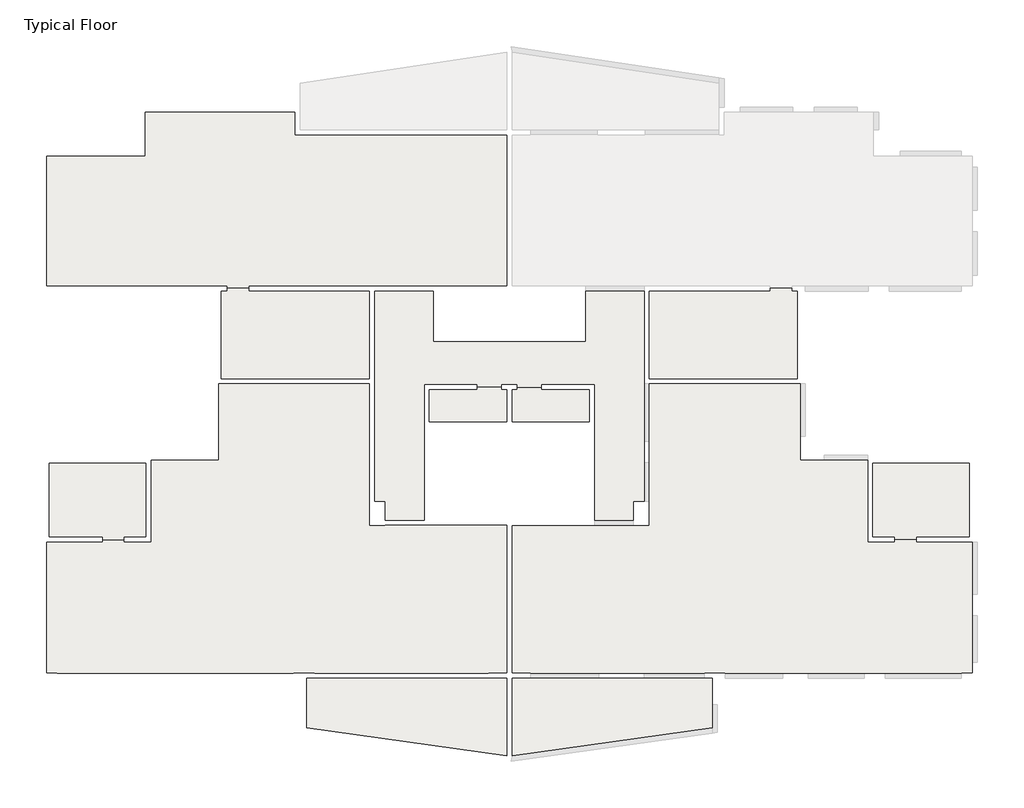
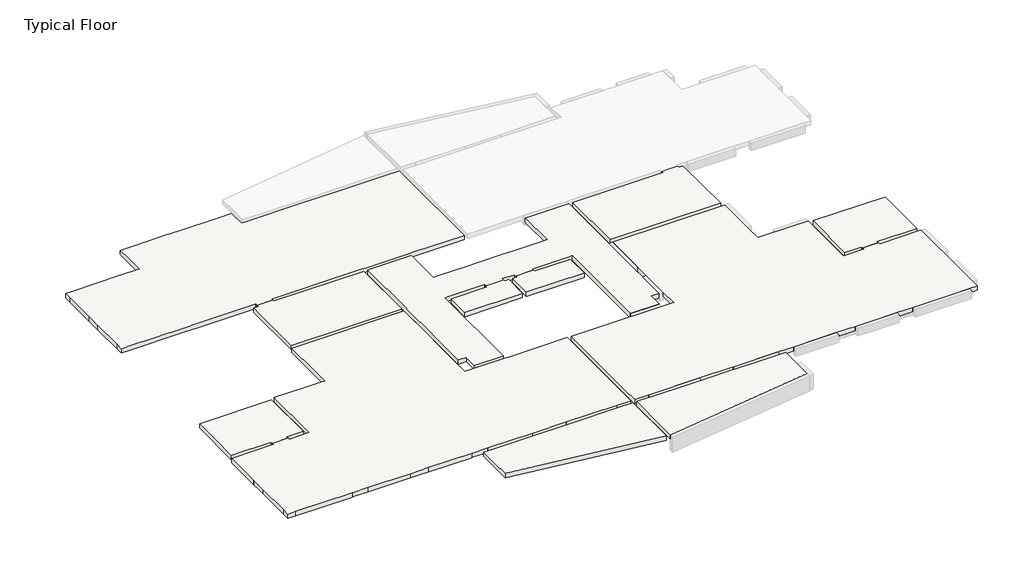
# One storey, part 1 of 2: 12 slabs.
"""IFC4 building model written with IfcOpenShell, lengths in millimetres."""

from ifc_helpers import new_model, si_unit, frame, origin, place, context, project, spatial, polyline, outline, extrude, faceted_brep, element, save

model = new_model("IFC4")

# Units and contexts
model_context = context("Model", 3, world=origin())
ifc_project = project(units=[si_unit("LENGTHUNIT", "METRE", prefix="MILLI")], contexts=[model_context])

# Site, building, storey
site = spatial("IfcSite", under=ifc_project)
building = spatial("IfcBuilding", under=site)
storey = spatial("IfcBuildingStorey", under=building, Name="Typical Floor", Elevation=3120.0)

# Slabs
placement = place(None, origin())
element("IfcSlab", 1, ObjectType="23", at=placement, inside=storey, context=model_context, shape_type="Brep", body=[
    faceted_brep([(-17867.839929, -8104.8146558, 2890.0), (-17867.839929, -8004.8146558, 2890.0), (-17067.8037495, -8004.8146558, 2890.0), (-17067.8037495, -8104.8146558, 2890.0), (-16045.535298, -8104.8146558, 2890.0), (-16045.535298, -7904.8146558, 2890.0), (-16045.535298, -5135.8928035, 2890.0), (-16045.535298, -5036.9600972, 2890.0), (-14415.271188, -5036.9600972, 2890.0), (-13515.271188, -5036.9600972, 2890.0), (-13515.271188, -4136.9600972, 2890.0), (-13515.271188, -2169.1055386, 2890.0), (-7866.3203921, -2169.1055386, 2890.0), (-7866.3023024, -7475.6540191, 2890.0), (-7266.3023024, -7475.6540191, 2890.0), (-7266.3023024, -7475.1655965, 2890.0), (-5816.5012893, -7475.1655965, 2890.0), (-5816.3023024, -7475.1655965, 2890.0), (-5616.5012893, -7475.1655965, 2890.0), (-2716.392751, -7475.1655965, 2890.0), (-2716.392751, -12204.5252202, 2890.0), (-2716.392751, -13004.5252202, 2890.0), (-3416.392751, -13004.5252202, 2890.0), (-3416.392751, -13009.5252202, 2890.0), (-5966.3203921, -13009.5252202, 2890.0), (-5966.3203921, -13005.5744243, 2890.0), (-6816.392751, -13005.5744243, 2890.0), (-7666.3203921, -13005.5744243, 2890.0), (-7666.3203921, -13009.5252202, 2890.0), (-9916.193764, -13009.5252202, 2890.0), (-9916.193764, -13004.5252202, 2890.0), (-10716.193764, -13004.5252202, 2890.0), (-10716.193764, -13009.5252202, 2890.0), (-12866.5555585, -13009.5252202, 2890.0), (-12866.5555585, -13005.8747137, 2890.0), (-13341.5555585, -13005.8747137, 2890.0), (-13816.5555585, -13005.8747137, 2890.0), (-13816.5555585, -13009.5252202, 2890.0), (-15916.4289304, -13009.5252202, 2890.0), (-15916.4289304, -13005.8747137, 2890.0), (-16316.4289304, -13005.8747137, 2890.0), (-16716.4289304, -13005.8747137, 2890.0), (-16716.4289304, -13009.5252202, 2890.0), (-19564.2400737, -13009.5252202, 2890.0), (-19564.2400737, -13004.5252202, 2890.0), (-19964.2400737, -13004.5252202, 2890.0), (-19964.2400737, -12604.5252202, 2890.0), (-19966.2400737, -12604.5252202, 2890.0), (-19966.2400737, -10855.1764503, 2890.0), (-19965.2892778, -10855.1764503, 2890.0), (-19965.2892778, -10455.1764503, 2890.0), (-19965.2892778, -10055.1764503, 2890.0), (-19966.2400737, -10055.1764503, 2890.0), (-19966.2400737, -8105.8819496, 2890.0), (-19964.2400737, -8105.8819496, 2890.0), (-19864.2400737, -8105.8819496, 2890.0), (-19864.2400737, -8104.8146558, 2890.0), (-17867.839929, -8004.8146558, 3120.0), (-17867.839929, -8104.8146558, 3120.0), (-19864.2400737, -8104.8146558, 3120.0), (-19864.2400737, -8105.8819496, 3120.0), (-19966.2400737, -8105.8819496, 3120.0), (-19966.2400737, -10055.1764503, 3120.0), (-19965.2892778, -10055.1764503, 3120.0), (-19965.2892778, -10855.1764503, 3120.0), (-19966.2400737, -10855.1764503, 3120.0), (-19966.2400737, -12604.5252202, 3120.0), (-19964.2400737, -12604.5252202, 3120.0), (-19964.2400737, -13004.5252202, 3120.0), (-19564.2400737, -13004.5252202, 3120.0), (-19564.2400737, -13009.5252202, 3120.0), (-16716.4289304, -13009.5252202, 3120.0), (-16716.4289304, -13005.8747137, 3120.0), (-15916.4289304, -13005.8747137, 3120.0), (-15916.4289304, -13009.5252202, 3120.0), (-13816.5555585, -13009.5252202, 3120.0), (-13816.5555585, -13005.8747137, 3120.0), (-12866.5555585, -13005.8747137, 3120.0), (-12866.5555585, -13009.5252202, 3120.0), (-10716.193764, -13009.5252202, 3120.0), (-10716.193764, -13004.5252202, 3120.0), (-9916.193764, -13004.5252202, 3120.0), (-9916.193764, -13009.5252202, 3120.0), (-7666.3203921, -13009.5252202, 3120.0), (-7666.3203921, -13005.5744243, 3120.0), (-5966.3203921, -13005.5744243, 3120.0), (-5966.3203921, -13009.5252202, 3120.0), (-3416.392751, -13009.5252202, 3120.0), (-3416.392751, -13004.5252202, 3120.0), (-2716.392751, -13004.5252202, 3120.0), (-2716.392751, -12204.5252202, 3120.0), (-2716.392751, -7475.1655965, 3120.0), (-5616.5012893, -7475.1655965, 3120.0), (-5816.5012893, -7475.1655965, 3120.0), (-7266.3023024, -7475.1655965, 3120.0), (-7266.3023024, -7475.6540191, 3120.0), (-7866.3023024, -7475.6540191, 3120.0), (-7866.3053704, -6575.654019, 3120.0), (-7866.3103273, -5121.5838309, 3120.0), (-7866.3130544, -4321.5838309, 3120.0), (-7866.3203921, -2169.1055386, 3120.0), (-13515.271188, -2169.1055386, 3120.0), (-13515.271188, -4136.9600972, 3120.0), (-13515.271188, -5036.9600972, 3120.0), (-14415.271188, -5036.9600972, 3120.0), (-16045.271188, -5036.9600972, 3120.0), (-16045.535298, -5036.9600972, 3120.0), (-16045.535298, -5135.8928035, 3120.0), (-16045.535298, -7904.8146558, 3120.0), (-16045.535298, -8104.8146558, 3120.0), (-17067.8037495, -8104.8146558, 3120.0), (-17067.8037495, -8004.8146558, 3120.0)], [[[0, 1, 2, 3, 4, 5, 6, 7, 8, 9, 10, 11, 12, 13, 14, 15, 16, 17, 18, 19, 20, 21, 22, 23, 24, 25, 26, 27, 28, 29, 30, 31, 32, 33, 34, 35, 36, 37, 38, 39, 40, 41, 42, 43, 44, 45, 46, 47, 48, 49, 50, 51, 52, 53, 54, 55, 56]], [[57, 58, 59, 60, 61, 62, 63, 64, 65, 66, 67, 68, 69, 70, 71, 72, 73, 74, 75, 76, 77, 78, 79, 80, 81, 82, 83, 84, 85, 86, 87, 88, 89, 90, 91, 92, 93, 94, 95, 96, 97, 98, 99, 100, 101, 102, 103, 104, 105, 106, 107, 108, 109, 110, 111]], [[12, 100, 99, 98, 97, 96, 13]], [[91, 19, 18, 17, 16, 15, 94, 93, 92]], [[19, 91, 90, 89, 21, 20]], [[23, 87, 86, 24]], [[82, 29, 28, 83]], [[32, 79, 78, 33]], [[70, 43, 42, 71]], [[74, 38, 37, 75]], [[47, 66, 65, 48]], [[61, 53, 52, 62]], [[58, 0, 56, 59]], [[1, 0, 58, 57]], [[2, 1, 57, 111]], [[3, 2, 111, 110]], [[4, 3, 110, 109]], [[4, 109, 108, 107, 106, 7, 6, 5]], [[7, 106, 105, 104, 103, 9, 8]], [[9, 103, 102, 101, 11, 10]], [[12, 11, 101, 100]], [[22, 88, 87, 23]], [[88, 22, 21, 89]], [[31, 80, 79, 32]], [[80, 31, 30, 81]], [[81, 30, 29, 82]], [[46, 67, 66, 47]], [[45, 68, 67, 46]], [[68, 45, 44, 69]], [[69, 44, 43, 70]], [[14, 95, 94, 15]], [[95, 14, 13, 96]], [[55, 60, 59, 56]], [[60, 55, 54, 53, 61]], [[49, 64, 63, 51, 50]], [[64, 49, 48, 65]], [[51, 63, 62, 52]], [[39, 73, 72, 41, 40]], [[73, 39, 38, 74]], [[41, 72, 71, 42]], [[34, 77, 76, 36, 35]], [[77, 34, 33, 78]], [[36, 76, 75, 37]], [[25, 85, 84, 27, 26]], [[85, 25, 24, 86]], [[27, 84, 83, 28]]]),
])
element("IfcSlab", 2, ObjectType="23", at=placement, inside=storey, context=model_context, shape_type="SweptSolid", body=[
    extrude(outline(polyline([(-16245.535298, -5135.8928035), (-16245.535298, -7904.8146558), (-17067.8037495, -7904.8146558), (-17067.8037495, -8004.8146558), (-17867.839929, -8004.8146558), (-17867.839929, -7904.8146558), (-19864.2400737, -7904.8146558), (-19864.2400737, -5135.8928035), (-16245.535298, -5135.8928035)])), frame((0.0, 0.0, 2890.0), z_axis=(0.0, 0.0, 1.0), x_axis=(1.0, 0.0, 0.0)), (0.0, 0.0, 1.0), 230.0),
])
element("IfcSlab", 3, ObjectType="23", at=placement, inside=storey, context=model_context, shape_type="Brep", body=[
    faceted_brep([(-2716.392751, -13204.5252202, 2890.0), (-2716.392751, -16112.674045, 2890.0), (-10216.193764, -15058.6457505, 2890.0), (-10216.193764, -14204.5252202, 2890.0), (-10216.193764, -13204.5252202, 2890.0), (-9916.193764, -13204.5252202, 2890.0), (-7666.3203921, -13204.5252202, 2890.0), (-7666.3203921, -13205.5744243, 2890.0), (-5966.3203921, -13205.5744243, 2890.0), (-5966.3203921, -13204.5252202, 2890.0), (-2716.392751, -16112.674045, 3120.0), (-2716.392751, -13204.5252202, 3120.0), (-3416.392751, -13204.5252202, 3120.0), (-5966.3203921, -13204.5252202, 3120.0), (-5966.3203921, -13205.5744243, 3120.0), (-7666.3203921, -13205.5744243, 3120.0), (-7666.3203921, -13204.5252202, 3120.0), (-9916.193764, -13204.5252202, 3120.0), (-10216.193764, -13204.5252202, 3120.0), (-10216.193764, -14204.5252202, 3120.0), (-10216.193764, -15058.6457505, 3120.0)], [[[0, 1, 2, 3, 4, 5, 6, 7, 8, 9]], [[10, 11, 12, 13, 14, 15, 16, 17, 18, 19, 20]], [[1, 0, 11, 10]], [[2, 1, 10, 20]], [[2, 20, 19, 18, 4, 3]], [[11, 0, 9, 13, 12]], [[4, 18, 17, 16, 6, 5]], [[8, 14, 13, 9]], [[14, 8, 7, 15]], [[15, 7, 6, 16]]]),
])
element("IfcSlab", 4, ObjectType="23", at=placement, inside=storey, context=model_context, shape_type="Brep", body=[
    faceted_brep([(-12396.6930404, 1513.6006842, 2890.0), (-12396.6930404, 1413.6006842, 2890.0), (-13195.271188, 1413.6006842, 2890.0), (-13196.6930404, 1413.6006842, 2890.0), (-13196.6930404, 1514.1252863, 2890.0), (-13715.271188, 1514.1252863, 2890.0), (-16062.5034601, 1514.1252863, 2890.0), (-16862.5034601, 1514.1252863, 2890.0), (-19564.2400737, 1514.1252863, 2890.0), (-19964.2400737, 1514.1252863, 2890.0), (-19964.2400737, 1914.1252863, 2890.0), (-19969.2400737, 1914.1252863, 2890.0), (-19969.2400737, 3539.1252863, 2890.0), (-19965.2892778, 3539.1252863, 2890.0), (-19965.2892778, 3934.6498883, 2890.0), (-19965.2892778, 4339.1252863, 2890.0), (-19969.2400737, 4339.1252863, 2890.0), (-19969.2400737, 5963.5645048, 2890.0), (-19964.2400737, 5963.5645048, 2890.0), (-19964.2400737, 6363.5645048, 2890.0), (-19564.2400737, 6363.5645048, 2890.0), (-17264.6018682, 6363.5645048, 2890.0), (-16264.6018682, 6363.5645048, 2890.0), (-16264.6018682, 7363.5645048, 2890.0), (-16264.6018682, 8012.3163138, 2890.0), (-11266.4470202, 8012.3163138, 2890.0), (-10666.4470202, 8012.3163138, 2890.0), (-10666.4470202, 7162.3163138, 2890.0), (-10466.4470202, 7162.3163138, 2890.0), (-10466.4470202, 7163.6006842, 2890.0), (-10466.4470202, 7163.7694287, 2890.0), (-7705.3941982, 7163.7694287, 2890.0), (-7705.3941982, 7163.6006842, 2890.0), (-5905.3941982, 7163.6006842, 2890.0), (-5905.3941982, 7163.7694287, 2890.0), (-3416.392751, 7163.7694287, 2890.0), (-3416.392751, 7163.6006842, 2890.0), (-2716.392751, 7163.6006842, 2890.0), (-2716.392751, 6363.6006842, 2890.0), (-2716.392751, 1513.6006842, 2890.0), (-5279.9781345, 1513.6006842, 2890.0), (-5479.9781345, 1513.6006842, 2890.0), (-7666.3203921, 1513.6006842, 2890.0), (-7866.3203921, 1513.6006842, 2890.0), (-12396.6930404, 1413.6006842, 3120.0), (-12396.6930404, 1513.6006842, 3120.0), (-7866.3203921, 1513.6006842, 3120.0), (-7666.3203921, 1513.6006842, 3120.0), (-5479.9781345, 1513.6006842, 3120.0), (-5279.9781345, 1513.6006842, 3120.0), (-2716.392751, 1513.6006842, 3120.0), (-2716.392751, 6363.6006842, 3120.0), (-2716.392751, 7163.6006842, 3120.0), (-3416.392751, 7163.6006842, 3120.0), (-3416.392751, 7163.7694287, 3120.0), (-5905.3941982, 7163.7694287, 3120.0), (-5905.3941982, 7163.6006842, 3120.0), (-7705.3941982, 7163.6006842, 3120.0), (-7705.3941982, 7163.7694287, 3120.0), (-10466.4470202, 7163.7694287, 3120.0), (-10466.4470202, 7162.3163138, 3120.0), (-10666.4470202, 7162.3163138, 3120.0), (-10666.4470202, 8012.3163138, 3120.0), (-11266.4470202, 8012.3163138, 3120.0), (-13239.0953559, 8012.3163138, 3120.0), (-14039.0953559, 8012.3163138, 3120.0), (-15664.5656888, 8012.3163138, 3120.0), (-16264.6018682, 8012.3163138, 3120.0), (-16264.6018682, 7363.5645048, 3120.0), (-16264.6018682, 6363.5645048, 3120.0), (-17264.6018682, 6363.5645048, 3120.0), (-19564.2400737, 6363.5645048, 3120.0), (-19964.2400737, 6363.5645048, 3120.0), (-19964.2400737, 5963.5645048, 3120.0), (-19969.2400737, 5963.5645048, 3120.0), (-19969.2400737, 4339.1252863, 3120.0), (-19965.2892778, 4339.1252863, 3120.0), (-19965.2892778, 3539.1252863, 3120.0), (-19969.2400737, 3539.1252863, 3120.0), (-19969.2400737, 1914.1252863, 3120.0), (-19964.2400737, 1914.1252863, 3120.0), (-19964.2400737, 1514.1252863, 3120.0), (-19564.2400737, 1514.1252863, 3120.0), (-16862.5034601, 1514.1252863, 3120.0), (-16062.5034601, 1514.1252863, 3120.0), (-13715.271188, 1514.1252863, 3120.0), (-13196.6930404, 1514.1252863, 3120.0), (-13196.6930404, 1413.6006842, 3120.0), (-13195.271188, 1413.6006842, 3120.0)], [[[0, 1, 2, 3, 4, 5, 6, 7, 8, 9, 10, 11, 12, 13, 14, 15, 16, 17, 18, 19, 20, 21, 22, 23, 24, 25, 26, 27, 28, 29, 30, 31, 32, 33, 34, 35, 36, 37, 38, 39, 40, 41, 42, 43]], [[44, 45, 46, 47, 48, 49, 50, 51, 52, 53, 54, 55, 56, 57, 58, 59, 60, 61, 62, 63, 64, 65, 66, 67, 68, 69, 70, 71, 72, 73, 74, 75, 76, 77, 78, 79, 80, 81, 82, 83, 84, 85, 86, 87, 88]], [[26, 62, 61, 27]], [[30, 59, 58, 31]], [[54, 35, 34, 55]], [[50, 39, 38, 37, 52, 51]], [[39, 50, 49, 48, 47, 46, 45, 0, 43, 42, 41, 40]], [[1, 0, 45, 44]], [[3, 2, 1, 44, 88, 87]], [[4, 3, 87, 86]], [[4, 86, 85, 84, 83, 82, 81, 9, 8, 7, 6, 5]], [[11, 79, 78, 12]], [[74, 17, 16, 75]], [[69, 22, 21, 20, 19, 72, 71, 70]], [[22, 69, 68, 67, 24, 23]], [[24, 67, 66, 65, 64, 63, 62, 26, 25]], [[36, 53, 52, 37]], [[53, 36, 35, 54]], [[10, 80, 79, 11]], [[80, 10, 9, 81]], [[18, 73, 72, 19]], [[73, 18, 17, 74]], [[28, 60, 59, 30, 29]], [[27, 61, 60, 28]], [[33, 56, 55, 34]], [[56, 33, 32, 57]], [[57, 32, 31, 58]], [[15, 76, 75, 16]], [[76, 15, 14, 13, 77]], [[77, 13, 12, 78]]]),
])
element("IfcSlab", 5, ObjectType="23", at=placement, inside=storey, context=model_context, shape_type="SweptSolid", body=[
    extrude(outline(polyline([(-7866.3203921, -1969.1055386), (-13415.271188, -1969.1055386), (-13415.271188, 1313.6006842), (-13195.271188, 1313.6006842), (-13195.271188, 1413.6006842), (-12396.6930404, 1413.6006842), (-12396.6930404, 1313.6006842), (-7866.3203921, 1313.6006842), (-7866.3203921, -1969.1055386)])), frame((0.0, 0.0, 2890.0), z_axis=(0.0, 0.0, 1.0), x_axis=(1.0, 0.0, 0.0)), (0.0, 0.0, 1.0), 230.0),
])
element("IfcSlab", 6, ObjectType="23", at=placement, inside=storey, context=model_context, shape_type="Brep", body=[
    faceted_brep([(11835.0182476, -8004.8146558, 2890.0), (12635.054427, -8004.8146558, 2890.0), (12635.054427, -8104.8146558, 2890.0), (14631.4545717, -8104.8146558, 2890.0), (14631.4545717, -8105.8819496, 2890.0), (14731.4545717, -8105.8819496, 2890.0), (14731.4545717, -12604.5252202, 2890.0), (14731.4545717, -13004.5252202, 2890.0), (14331.4545717, -13004.5252202, 2890.0), (14331.4545717, -13009.5252202, 2890.0), (11483.6434285, -13009.5252202, 2890.0), (11483.6434285, -13005.8747137, 2890.0), (11083.6434285, -13005.8747137, 2890.0), (10683.6434285, -13005.8747137, 2890.0), (10683.6434285, -13009.5252202, 2890.0), (8583.7700565, -13009.5252202, 2890.0), (8583.7700565, -13005.8747137, 2890.0), (8108.7700565, -13005.8747137, 2890.0), (7633.7700565, -13005.8747137, 2890.0), (7633.7700565, -13009.5252202, 2890.0), (5483.408262, -13009.5252202, 2890.0), (5483.408262, -13004.5252202, 2890.0), (4683.408262, -13004.5252202, 2890.0), (4683.408262, -13009.5252202, 2890.0), (2433.5348901, -13009.5252202, 2890.0), (2433.5348901, -13005.5744243, 2890.0), (1583.607249, -13005.5744243, 2890.0), (733.5348901, -13005.5744243, 2890.0), (733.5348901, -13009.5252202, 2890.0), (-1816.392751, -13009.5252202, 2890.0), (-1816.392751, -13004.5252202, 2890.0), (-2516.392751, -13004.5252202, 2890.0), (-2516.392751, -12204.5252202, 2890.0), (-2516.392751, -7475.6540191, 2890.0), (2033.5168004, -7475.6540191, 2890.0), (2633.5348901, -7475.6540191, 2890.0), (2633.5348901, -6575.6540191, 2890.0), (2633.5348901, -5121.583831, 2890.0), (2633.5348901, -4321.583831, 2890.0), (2633.5348901, -2169.1055386, 2890.0), (8282.4856861, -2169.1055386, 2890.0), (8282.4856861, -4136.9600972, 2890.0), (8282.4856861, -5036.9600972, 2890.0), (9182.4856861, -5036.9600972, 2890.0), (10812.749796, -5036.9600972, 2890.0), (10812.749796, -5135.8928035, 2890.0), (10812.749796, -7904.8146558, 2890.0), (10812.749796, -8104.8146558, 2890.0), (11835.0182476, -8104.8146558, 2890.0), (12635.054427, -8004.8146558, 3120.0), (11835.0182476, -8004.8146558, 3120.0), (11835.0182476, -8104.8146558, 3120.0), (10812.749796, -8104.8146558, 3120.0), (10812.749796, -7904.8146558, 3120.0), (10812.749796, -5135.8928035, 3120.0), (10812.749796, -5036.9600972, 3120.0), (10812.4856861, -5036.9600972, 3120.0), (9182.4856861, -5036.9600972, 3120.0), (8282.4856861, -5036.9600972, 3120.0), (8282.4856861, -4136.9600972, 3120.0), (8282.4856861, -2169.1055386, 3120.0), (2633.5348901, -2169.1055386, 3120.0), (2633.5348901, -4321.583831, 3120.0), (2633.5348901, -5121.583831, 3120.0), (2633.5348901, -6575.6540191, 3120.0), (2633.5348901, -7475.6540191, 3120.0), (2033.5168004, -7475.6540191, 3120.0), (583.5168004, -7475.6540191, 3120.0), (-2516.392751, -7475.6540191, 3120.0), (-2516.392751, -12204.5252202, 3120.0), (-2516.392751, -13004.5252202, 3120.0), (-1816.392751, -13004.5252202, 3120.0), (-1816.392751, -13009.5252202, 3120.0), (733.5348901, -13009.5252202, 3120.0), (733.5348901, -13005.5744243, 3120.0), (2433.5348901, -13005.5744243, 3120.0), (2433.5348901, -13009.5252202, 3120.0), (4683.408262, -13009.5252202, 3120.0), (4683.408262, -13004.5252202, 3120.0), (5483.408262, -13004.5252202, 3120.0), (5483.408262, -13009.5252202, 3120.0), (7633.7700565, -13009.5252202, 3120.0), (7633.7700565, -13005.8747137, 3120.0), (8583.7700565, -13005.8747137, 3120.0), (8583.7700565, -13009.5252202, 3120.0), (10683.6434285, -13009.5252202, 3120.0), (10683.6434285, -13005.8747137, 3120.0), (11483.6434285, -13005.8747137, 3120.0), (11483.6434285, -13009.5252202, 3120.0), (14331.4545717, -13009.5252202, 3120.0), (14331.4545717, -13004.5252202, 3120.0), (14731.4545717, -13004.5252202, 3120.0), (14731.4545717, -12604.5252202, 3120.0), (14731.4545717, -10455.1764503, 3120.0), (14731.4545717, -8105.8819496, 3120.0), (14631.4545717, -8105.8819496, 3120.0), (14631.4545717, -8104.8146558, 3120.0), (12635.054427, -8104.8146558, 3120.0)], [[[0, 1, 2, 3, 4, 5, 6, 7, 8, 9, 10, 11, 12, 13, 14, 15, 16, 17, 18, 19, 20, 21, 22, 23, 24, 25, 26, 27, 28, 29, 30, 31, 32, 33, 34, 35, 36, 37, 38, 39, 40, 41, 42, 43, 44, 45, 46, 47, 48]], [[49, 50, 51, 52, 53, 54, 55, 56, 57, 58, 59, 60, 61, 62, 63, 64, 65, 66, 67, 68, 69, 70, 71, 72, 73, 74, 75, 76, 77, 78, 79, 80, 81, 82, 83, 84, 85, 86, 87, 88, 89, 90, 91, 92, 93, 94, 95, 96, 97]], [[35, 65, 64, 63, 62, 61, 39, 38, 37, 36]], [[33, 68, 67, 66, 65, 35, 34]], [[68, 33, 32, 31, 70, 69]], [[72, 29, 28, 73]], [[23, 77, 76, 24]], [[80, 20, 19, 81]], [[9, 89, 88, 10]], [[14, 85, 84, 15]], [[91, 7, 6, 5, 94, 93, 92]], [[1, 49, 97, 2]], [[1, 0, 50, 49]], [[0, 48, 51, 50]], [[48, 47, 52, 51]], [[44, 55, 54, 53, 52, 47, 46, 45]], [[42, 58, 57, 56, 55, 44, 43]], [[40, 60, 59, 58, 42, 41]], [[40, 39, 61, 60]], [[30, 71, 70, 31]], [[71, 30, 29, 72]], [[79, 21, 20, 80]], [[21, 79, 78, 22]], [[22, 78, 77, 23]], [[90, 8, 7, 91]], [[8, 90, 89, 9]], [[95, 4, 3, 96]], [[4, 95, 94, 5]], [[2, 97, 96, 3]], [[86, 13, 12, 11, 87]], [[13, 86, 85, 14]], [[87, 11, 10, 88]], [[82, 18, 17, 16, 83]], [[18, 82, 81, 19]], [[83, 16, 15, 84]], [[74, 27, 26, 25, 75]], [[27, 74, 73, 28]], [[75, 25, 24, 76]]]),
])
element("IfcSlab", 7, ObjectType="23", at=placement, inside=storey, context=model_context, shape_type="SweptSolid", body=[
    extrude(outline(polyline([(11012.749796, -7904.8146558), (11012.749796, -5135.8928035), (14631.4545717, -5135.8928035), (14631.4545717, -7904.8146558), (12635.054427, -7904.8146558), (12635.054427, -8004.8146558), (11835.0182476, -8004.8146558), (11835.0182476, -7904.8146558), (11012.749796, -7904.8146558)])), frame((0.0, 0.0, 2890.0), z_axis=(0.0, 0.0, 1.0), x_axis=(1.0, 0.0, 0.0)), (0.0, 0.0, 1.0), 230.0),
])
element("IfcSlab", 8, ObjectType="23", at=placement, inside=storey, context=model_context, shape_type="Brep", body=[
    faceted_brep([(-2516.392751, -16112.674045, 2890.0), (-2516.392751, -13204.5252202, 2890.0), (733.5348901, -13204.5252202, 2890.0), (733.5348901, -13205.5744243, 2890.0), (2433.5348901, -13205.5744243, 2890.0), (2433.5348901, -13204.5252202, 2890.0), (4683.408262, -13204.5252202, 2890.0), (4983.408262, -13204.5252202, 2890.0), (4983.408262, -14204.5252202, 2890.0), (4983.408262, -15058.6457505, 2890.0), (-2516.392751, -13204.5252202, 3120.0), (-2516.392751, -16112.674045, 3120.0), (4983.408262, -15058.6457505, 3120.0), (4983.408262, -14204.5252202, 3120.0), (4983.408262, -13204.5252202, 3120.0), (4683.408262, -13204.5252202, 3120.0), (2433.5348901, -13204.5252202, 3120.0), (2433.5348901, -13205.5744243, 3120.0), (733.5348901, -13205.5744243, 3120.0), (733.5348901, -13204.5252202, 3120.0), (-1816.392751, -13204.5252202, 3120.0)], [[[0, 1, 2, 3, 4, 5, 6, 7, 8, 9]], [[10, 11, 12, 13, 14, 15, 16, 17, 18, 19, 20]], [[1, 0, 11, 10]], [[0, 9, 12, 11]], [[7, 14, 13, 12, 9, 8]], [[1, 10, 20, 19, 2]], [[14, 7, 6, 5, 16, 15]], [[18, 3, 2, 19]], [[3, 18, 17, 4]], [[4, 17, 16, 5]]]),
])
element("IfcSlab", 9, ObjectType="23", at=placement, inside=storey, context=model_context, shape_type="SweptSolid", body=[
    extrude(outline(polyline([(8182.4856861, -1969.1055386), (2633.5348901, -1969.1055386), (2633.5348901, 1313.6006842), (7163.9075385, 1313.6006842), (7163.9075385, 1413.6006842), (7962.4856861, 1413.6006842), (7962.4856861, 1313.6006842), (8182.4856861, 1313.6006842), (8182.4856861, -1969.1055386)])), frame((0.0, 0.0, 2890.0), z_axis=(0.0, 0.0, 1.0), x_axis=(1.0, 0.0, 0.0)), (0.0, 0.0, 1.0), 230.0),
])
element("IfcSlab", 10, ObjectType="23", at=placement, inside=storey, context=model_context, shape_type="Brep", body=[
    faceted_brep([(-5479.9781345, 1313.6006842, 2890.0), (-5479.9781345, -585.9651624, 2890.0), (-5279.9781345, -585.9651624, 2890.0), (-3638.6250231, -585.9651624, 2890.0), (-3438.6250231, -585.9651624, 2890.0), (-1794.1604789, -585.9651624, 2890.0), (-1594.1604789, -585.9651624, 2890.0), (47.1926325, -585.9651624, 2890.0), (247.1926325, -585.9651624, 2890.0), (247.1926325, 1313.6006842, 2890.0), (2433.5348901, 1313.6006842, 2890.0), (2433.5348901, -6575.6540191, 2890.0), (2033.5168004, -6575.6540191, 2890.0), (2033.5168004, -7275.6540191, 2890.0), (583.7157874, -7275.6540191, 2890.0), (583.7157874, -2183.9210234, 2890.0), (383.7157874, -2183.9210234, 2890.0), (-1416.3746613, -2183.9210234, 2890.0), (-1416.3746613, -2283.9210234, 2890.0), (-1419.486094, -2283.9210234, 2890.0), (-2315.8862387, -2283.9210234, 2890.0), (-2315.8862387, -2183.9210234, 2890.0), (-2916.8992633, -2183.9210234, 2890.0), (-2916.8992633, -2283.9210234, 2890.0), (-3816.4108407, -2283.9210234, 2890.0), (-3816.4108407, -2183.9210234, 2890.0), (-5616.5012893, -2183.9210234, 2890.0), (-5816.5012893, -2183.9210234, 2890.0), (-5816.5012893, -7275.6540191, 2890.0), (-7266.3023024, -7275.6540191, 2890.0), (-7266.3023024, -6575.6540191, 2890.0), (-7666.3203921, -6575.6540191, 2890.0), (-7666.3203921, 1313.6006842, 2890.0), (-5479.9781345, -585.9651624, 3120.0), (-5479.9781345, 1313.6006842, 3120.0), (-7666.3203921, 1313.6006842, 3120.0), (-7666.3203921, -1969.1055386, 3120.0), (-7666.3203921, -2169.1055386, 3120.0), (-7666.3203921, -4321.583831, 3120.0), (-7666.3203921, -5121.583831, 3120.0), (-7666.3203921, -6575.6540191, 3120.0), (-7266.3023024, -6575.6540191, 3120.0), (-7266.3023024, -7275.6540191, 3120.0), (-5816.5012893, -7275.6540191, 3120.0), (-5816.5012893, -2183.9210234, 3120.0), (-5616.5012893, -2183.9210234, 3120.0), (-3816.4108407, -2183.9210234, 3120.0), (-3816.4108407, -2283.9210234, 3120.0), (-2916.8992633, -2283.9210234, 3120.0), (-2916.8992633, -2183.9210234, 3120.0), (-2315.8862387, -2183.9210234, 3120.0), (-2315.8862387, -2283.9210234, 3120.0), (-1419.486094, -2283.9210234, 3120.0), (-1416.3746613, -2283.9210234, 3120.0), (-1416.3746613, -2183.9210234, 3120.0), (383.7157874, -2183.9210234, 3120.0), (583.7157874, -2183.9210234, 3120.0), (583.7157874, -7275.6540191, 3120.0), (2033.5168004, -7275.6540191, 3120.0), (2033.5168004, -6575.6540191, 3120.0), (2433.5348901, -6575.6540191, 3120.0), (2433.5348901, -5121.583831, 3120.0), (2433.5348901, -4321.583831, 3120.0), (2433.5348901, -2169.1055386, 3120.0), (2433.5348901, -1969.1055386, 3120.0), (2433.5348901, 1313.6006842, 3120.0), (247.1926325, 1313.6006842, 3120.0), (247.1926325, -585.9651624, 3120.0), (47.1926325, -585.9651624, 3120.0), (-1594.1604789, -585.9651624, 3120.0), (-1794.1604789, -585.9651624, 3120.0), (-3438.6250231, -585.9651624, 3120.0), (-3638.6250231, -585.9651624, 3120.0), (-5279.9781345, -585.9651624, 3120.0)], [[[0, 1, 2, 3, 4, 5, 6, 7, 8, 9, 10, 11, 12, 13, 14, 15, 16, 17, 18, 19, 20, 21, 22, 23, 24, 25, 26, 27, 28, 29, 30, 31, 32]], [[33, 34, 35, 36, 37, 38, 39, 40, 41, 42, 43, 44, 45, 46, 47, 48, 49, 50, 51, 52, 53, 54, 55, 56, 57, 58, 59, 60, 61, 62, 63, 64, 65, 66, 67, 68, 69, 70, 71, 72, 73]], [[1, 0, 34, 33]], [[1, 33, 73, 72, 71, 70, 69, 68, 67, 8, 7, 6, 5, 4, 3, 2]], [[9, 8, 67, 66]], [[10, 9, 66, 65]], [[11, 10, 65, 64, 63, 62, 61, 60]], [[12, 11, 60, 59]], [[13, 12, 59, 58]], [[14, 13, 58, 57]], [[15, 14, 57, 56]], [[15, 56, 55, 54, 17, 16]], [[18, 17, 54, 53]], [[20, 19, 18, 53, 52, 51]], [[21, 20, 51, 50]], [[22, 21, 50, 49]], [[23, 22, 49, 48]], [[24, 23, 48, 47]], [[25, 24, 47, 46]], [[25, 46, 45, 44, 27, 26]], [[28, 27, 44, 43]], [[29, 28, 43, 42]], [[30, 29, 42, 41]], [[31, 30, 41, 40]], [[32, 31, 40, 39, 38, 37, 36, 35]], [[0, 32, 35, 34]]]),
])
element("IfcSlab", 11, ObjectType="23", at=placement, inside=storey, context=model_context, shape_type="SweptSolid", body=[
    extrude(outline(polyline([(-3816.4108407, -2383.9210234), (-3816.4108407, -2283.9210234), (-2916.8992633, -2283.9210234), (-2916.8992633, -2383.9210234), (-2717.9484673, -2383.9210234), (-2717.9484673, -3585.0425864), (-5616.5012893, -3585.0425864), (-5616.5012893, -2383.9210234), (-3816.4108407, -2383.9210234)])), frame((0.0, 0.0, 2890.0), z_axis=(0.0, 0.0, 1.0), x_axis=(1.0, 0.0, 0.0)), (0.0, 0.0, 1.0), 230.0),
])
element("IfcSlab", 12, ObjectType="23", at=placement, inside=storey, context=model_context, shape_type="Brep", body=[
    faceted_brep([(-1419.486094, -2283.9210234, 2890.0), (-1419.486094, -2383.9210234, 2890.0), (-1416.3746613, -2383.9210234, 2890.0), (383.7157874, -2383.9210234, 2890.0), (383.7157874, -3585.0425864, 2890.0), (-2517.9484673, -3585.0425864, 2890.0), (-2517.9484673, -2383.9210234, 2890.0), (-2315.8862387, -2383.9210234, 2890.0), (-2315.8862387, -2283.9210234, 2890.0), (-1419.486094, -2383.9210234, 3120.0), (-1419.486094, -2283.9210234, 3120.0), (-2315.8862387, -2283.9210234, 3120.0), (-2315.8862387, -2383.9210234, 3120.0), (-2517.9484673, -2383.9210234, 3120.0), (-2517.9484673, -3585.0425864, 3120.0), (383.7157874, -3585.0425864, 3120.0), (383.7157874, -2383.9210234, 3120.0), (-1416.3746613, -2383.9210234, 3120.0)], [[[0, 1, 2, 3, 4, 5, 6, 7, 8]], [[9, 10, 11, 12, 13, 14, 15, 16, 17]], [[14, 5, 4, 15]], [[1, 9, 17, 16, 3, 2]], [[1, 0, 10, 9]], [[0, 8, 11, 10]], [[8, 7, 12, 11]], [[7, 6, 13, 12]], [[6, 5, 14, 13]], [[4, 3, 16, 15]]]),
])

save(model, "model.ifc")

# Revit data of these elements
# Type "23"
#   Function = 0
#   Layers, outside or top first: 23 cm "Concrete" (function 1)
# Element 1 (IfcSlab, "23")
#   Mark = "S1"
#   SOFiSTiK_AMG_Comments = ""
#   Height Offset From Level = 0 cm
#   built-in parameter 1001954 = 1
#   SOFiSTiK_AMG_Scheduled = yes
#   SOFiSTiK_AMG_Adjusted = yes
#   Phase Created = New Construction
#   Materials on its faces: "Concrete"
# Element 2 (IfcSlab, "23")
#   Mark = "S2"
#   SOFiSTiK_AMG_Comments = ""
#   Height Offset From Level = 0 cm
#   built-in parameter 1001954 = 1
#   SOFiSTiK_AMG_Scheduled = yes
#   SOFiSTiK_AMG_Adjusted = yes
#   Phase Created = New Construction
#   Materials on its faces: "Concrete"
# Element 3 (IfcSlab, "23")
#   Mark = "S3"
#   SOFiSTiK_AMG_Comments = ""
#   Height Offset From Level = 0 cm
#   built-in parameter 1001954 = 1
#   SOFiSTiK_AMG_Scheduled = yes
#   SOFiSTiK_AMG_Adjusted = yes
#   Phase Created = New Construction
#   Materials on its faces: "Concrete"
# Element 4 (IfcSlab, "23")
#   Mark = "S4"
#   SOFiSTiK_AMG_Comments = ""
#   Height Offset From Level = 0 cm
#   built-in parameter 1001954 = 1
#   SOFiSTiK_AMG_Scheduled = yes
#   SOFiSTiK_AMG_Adjusted = yes
#   Phase Created = New Construction
#   Materials on its faces: "Concrete"
# Element 5 (IfcSlab, "23")
#   Mark = "S5"
#   SOFiSTiK_AMG_Comments = ""
#   Height Offset From Level = 0 cm
#   built-in parameter 1001954 = 1
#   SOFiSTiK_AMG_Scheduled = yes
#   SOFiSTiK_AMG_Adjusted = yes
#   Phase Created = New Construction
#   Materials on its faces: "Concrete"
# Element 6 (IfcSlab, "23")
#   Mark = "S7"
#   SOFiSTiK_AMG_Comments = ""
#   built-in parameter 1001955 = 3.14159 (stored number, unit not read)
#   Height Offset From Level = 0 cm
#   built-in parameter 1001954 = 1
#   SOFiSTiK_AMG_Scheduled = yes
#   SOFiSTiK_AMG_Adjusted = yes
#   Phase Created = New Construction
#   Materials on its faces: "Concrete"
# Element 7 (IfcSlab, "23")
#   Mark = "S8"
#   SOFiSTiK_AMG_Comments = ""
#   built-in parameter 1001955 = 3.14159 (stored number, unit not read)
#   Height Offset From Level = 0 cm
#   built-in parameter 1001954 = 1
#   SOFiSTiK_AMG_Scheduled = yes
#   SOFiSTiK_AMG_Adjusted = yes
#   Phase Created = New Construction
#   Materials on its faces: "Concrete"
# Element 8 (IfcSlab, "23")
#   Mark = "S9"
#   SOFiSTiK_AMG_Comments = ""
#   built-in parameter 1001955 = 3.14159 (stored number, unit not read)
#   Height Offset From Level = 0 cm
#   built-in parameter 1001954 = 1
#   SOFiSTiK_AMG_Scheduled = yes
#   SOFiSTiK_AMG_Adjusted = yes
#   Phase Created = New Construction
#   Materials on its faces: "Concrete"
# Element 9 (IfcSlab, "23")
#   Mark = "S11"
#   SOFiSTiK_AMG_Comments = ""
#   built-in parameter 1001955 = 3.14159 (stored number, unit not read)
#   Height Offset From Level = 0 cm
#   built-in parameter 1001954 = 1
#   SOFiSTiK_AMG_Scheduled = yes
#   SOFiSTiK_AMG_Adjusted = yes
#   Phase Created = New Construction
#   Materials on its faces: "Concrete"
# Element 10 (IfcSlab, "23")
#   Mark = "S13"
#   SOFiSTiK_AMG_Comments = ""
#   Height Offset From Level = 0 cm
#   built-in parameter 1001954 = 1
#   SOFiSTiK_AMG_Scheduled = yes
#   SOFiSTiK_AMG_Adjusted = yes
#   Phase Created = New Construction
#   Materials on its faces: "Concrete"
# Element 11 (IfcSlab, "23")
#   Mark = "S14"
#   SOFiSTiK_AMG_Comments = ""
#   Height Offset From Level = 0 cm
#   built-in parameter 1001954 = 1
#   SOFiSTiK_AMG_Scheduled = yes
#   SOFiSTiK_AMG_Adjusted = yes
#   Phase Created = New Construction
#   Materials on its faces: "Concrete"
# Element 12 (IfcSlab, "23")
#   Mark = "S15"
#   SOFiSTiK_AMG_Comments = ""
#   built-in parameter 1001955 = 3.14159 (stored number, unit not read)
#   Height Offset From Level = 0 cm
#   built-in parameter 1001954 = 1
#   SOFiSTiK_AMG_Scheduled = yes
#   SOFiSTiK_AMG_Adjusted = yes
#   Phase Created = New Construction
#   Materials on its faces: "Concrete"
# Materials
#   "Concrete": class "Concrete", colour RGB 192 192 192, transparency 0, Keynote = "01000", Description = "Cast-in-place concrete", Cost = 0
